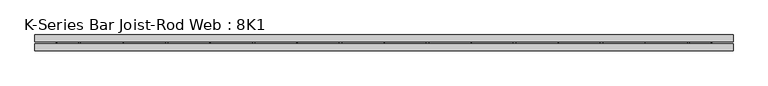
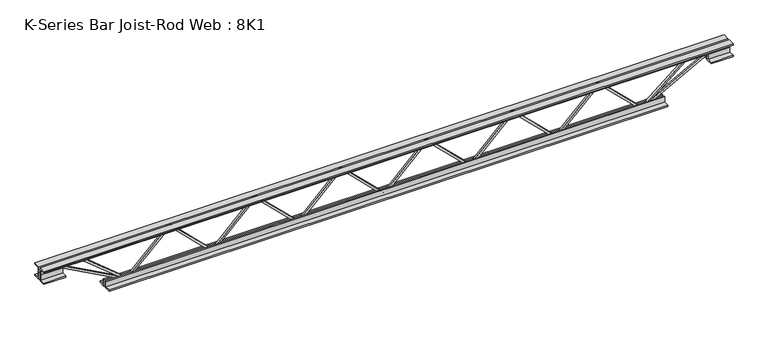
"""IFC4 building model written with IfcOpenShell, lengths in millimetres: beam geometry, K-Series Bar Joist-Rod Web : 8K1."""

from ifc_helpers import new_model, si_unit, frame, origin, place, context, project, spatial, polyline, outline, extrude, source, transform, mapped, element, save


def k_series_bar_joist_rod_web_8k1_a6564055(model_context):
    return source(origin(), model_context, "Body", "SweptSolid", [
        extrude(outline(polyline([(-90.4875, 401.8896924), (-100.0125, 401.8896924), (-100.0125, 407.0077855), (90.4875, 601.6026317), (90.4875, 604.0664455), (-100.0125, 798.6612917), (-100.0125, 803.7793848), (-90.4875, 803.7793848), (-90.4875, 802.5474779), (100.0125, 607.9526317), (100.0125, 597.7164455), (-90.4875, 403.1215993), (-90.4875, 401.8896924)])), frame((0.0, -4.7625, 0.0), z_axis=(0.0, 1.0, 0.0), x_axis=(0.0, 0.0, 1.0)), (0.0, 0.0, 1.0), 9.525),
        extrude(outline(polyline([(-90.4875, 0.0), (-100.0125, 0.0), (-100.0125, 5.1180931), (90.4875, 199.7129393), (90.4875, 202.1767531), (-100.0125, 396.7715993), (-100.0125, 401.8896924), (-90.4875, 401.8896924), (-90.4875, 400.6577855), (100.0125, 206.0629393), (100.0125, 195.8267531), (-90.4875, 1.2319069), (-90.4875, 0.0)])), frame((0.0, -4.7625, 0.0), z_axis=(0.0, 1.0, 0.0), x_axis=(0.0, 0.0, 1.0)), (0.0, 0.0, 1.0), 9.525),
        extrude(outline(polyline([(-90.4875, -401.8896924), (-100.0125, -401.8896924), (-100.0125, -396.7715993), (90.4875, -202.1767531), (90.4875, -199.7129393), (-100.0125, -5.1180931), (-100.0125, 0.0), (-90.4875, 0.0), (-90.4875, -1.2319069), (100.0125, -195.8267531), (100.0125, -206.0629393), (-90.4875, -400.6577855), (-90.4875, -401.8896924)])), frame((0.0, -4.7625, 0.0), z_axis=(0.0, 1.0, 0.0), x_axis=(0.0, 0.0, 1.0)), (0.0, 0.0, 1.0), 9.525),
        extrude(outline(polyline([(-90.4875, -803.7793848), (-100.0125, -803.7793848), (-100.0125, -798.6612917), (90.4875, -604.0664455), (90.4875, -601.6026317), (-100.0125, -407.0077855), (-100.0125, -401.8896924), (-90.4875, -401.8896924), (-90.4875, -403.1215993), (100.0125, -597.7164455), (100.0125, -607.9526317), (-90.4875, -802.5474779), (-90.4875, -803.7793848)])), frame((0.0, -4.7625, 0.0), z_axis=(0.0, 1.0, 0.0), x_axis=(0.0, 0.0, 1.0)), (0.0, 0.0, 1.0), 9.525),
        extrude(outline(polyline([(-90.4875, 803.7793848), (-100.0125, 803.7793848), (-100.0125, 808.8974779), (90.4875, 1003.4923241), (90.4875, 1005.9561379), (-100.0125, 1200.5509841), (-100.0125, 1205.6690772), (-90.4875, 1205.6690772), (-90.4875, 1204.4371703), (100.0125, 1009.8423241), (100.0125, 999.6061379), (-90.4875, 805.0112917), (-90.4875, 803.7793848)])), frame((0.0, -4.7625, 0.0), z_axis=(0.0, 1.0, 0.0), x_axis=(0.0, 0.0, 1.0)), (0.0, 0.0, 1.0), 9.525),
        extrude(outline(polyline([(-90.4875, -1205.6690772), (-100.0125, -1205.6690772), (-100.0125, -1200.5509841), (90.4875, -1005.9561379), (90.4875, -1003.4923241), (-100.0125, -808.8974779), (-100.0125, -803.7793848), (-90.4875, -803.7793848), (-90.4875, -805.0112917), (100.0125, -999.6061379), (100.0125, -1009.8423241), (-90.4875, -1204.4371703), (-90.4875, -1205.6690772)])), frame((0.0, -4.7625, 0.0), z_axis=(0.0, 1.0, 0.0), x_axis=(0.0, 0.0, 1.0)), (0.0, 0.0, 1.0), 9.525),
        extrude(outline(polyline([(4.7625, 101.6), (36.5125, 101.6), (36.5125, 95.25), (11.1125, 95.25), (11.1125, 69.85), (4.7625, 69.85), (4.7625, 101.6)])), frame((-1612.0690772, 0.0, 0.0), z_axis=(1.0, 0.0, 0.0), x_axis=(0.0, 1.0, 0.0)), (0.0, 0.0, 1.0), 3224.1381544),
        extrude(outline(polyline([(-4.7625, 101.6), (-4.7625, 69.85), (-11.1125, 69.85), (-11.1125, 95.25), (-36.5125, 95.25), (-36.5125, 101.6), (-4.7625, 101.6)])), frame((-1612.0690772, 0.0, 0.0), z_axis=(1.0, 0.0, 0.0), x_axis=(0.0, 1.0, 0.0)), (0.0, 0.0, 1.0), 3224.1381544),
        extrude(outline(polyline([(-4.7625, 38.1), (-36.5125, 38.1), (-36.5125, 44.45), (-11.1125, 44.45), (-11.1125, 69.85), (-4.7625, 69.85), (-4.7625, 38.1)])), frame((-1612.0690772, 0.0, 0.0), z_axis=(1.0, 0.0, 0.0), x_axis=(0.0, 1.0, 0.0)), (0.0, 0.0, 1.0), 101.6),
        extrude(outline(polyline([(36.5125, 38.1), (4.7625, 38.1), (4.7625, 69.85), (11.1125, 69.85), (11.1125, 44.45), (36.5125, 44.45), (36.5125, 38.1)])), frame((-1612.0690772, 0.0, 0.0), z_axis=(1.0, 0.0, 0.0), x_axis=(0.0, 1.0, 0.0)), (0.0, 0.0, 1.0), 101.6),
        extrude(outline(polyline([(4.7625, 38.1), (4.7625, 69.85), (11.1125, 69.85), (11.1125, 44.45), (36.5125, 44.45), (36.5125, 38.1), (4.7625, 38.1)])), frame((1510.4690772, 0.0, 0.0), z_axis=(1.0, 0.0, 0.0), x_axis=(0.0, 1.0, 0.0)), (0.0, 0.0, 1.0), 101.6),
        extrude(outline(polyline([(-4.7625, 38.1), (-36.5125, 38.1), (-36.5125, 44.45), (-11.1125, 44.45), (-11.1125, 69.85), (-4.7625, 69.85), (-4.7625, 38.1)])), frame((1510.4690772, 0.0, 0.0), z_axis=(1.0, 0.0, 0.0), x_axis=(0.0, 1.0, 0.0)), (0.0, 0.0, 1.0), 101.6),
        extrude(outline(polyline([(4.7625, -101.6), (4.7625, -69.85), (11.1125, -69.85), (11.1125, -95.25), (36.5125, -95.25), (36.5125, -101.6), (4.7625, -101.6)])), frame((-1307.2690772, 0.0, 0.0), z_axis=(1.0, 0.0, 0.0), x_axis=(0.0, 1.0, 0.0)), (0.0, 0.0, 1.0), 2614.5381544),
        extrude(outline(polyline([(-4.7625, -101.6), (-36.5125, -101.6), (-36.5125, -95.25), (-11.1125, -95.25), (-11.1125, -69.85), (-4.7625, -69.85), (-4.7625, -101.6)])), frame((-1307.2690772, 0.0, 0.0), z_axis=(1.0, 0.0, 0.0), x_axis=(0.0, 1.0, 0.0)), (0.0, 0.0, 1.0), 2614.5381544),
        extrude(outline(polyline([(0.0, -9.525), (0.0, 0.0), (346.6425392, 0.0), (346.6425392, -9.525), (0.0, -9.525)])), frame((-1512.7373757, 4.7625, 65.662372), z_axis=(0.47628314854007997, 0.0, 0.8792919665371384), x_axis=(0.8792919665371384, 0.0, -0.47628314854007997)), (0.0, 0.0, 1.0), 9.525),
        extrude(outline(polyline([(0.0, -9.525), (0.0, 0.0), (260.0708388, 0.0), (260.0708388, -9.525), (0.0, -9.525)])), frame((-1409.6372872, 4.7625, 66.170234), z_axis=(0.6348270368814928, 0.0, 0.7726542779563599), x_axis=(0.7726542779563599, 0.0, -0.6348270368814928)), (0.0, 0.0, 1.0), 9.525),
        extrude(outline(polyline([(0.0, -9.525), (0.0, 0.0), (346.6425392, 0.0), (346.6425392, -9.525), (0.0, -9.525)])), frame((1512.7373757, -4.7625, 65.662372), z_axis=(-0.4762831485400427, 0.0, 0.8792919665371586), x_axis=(-0.8792919665371586, 0.0, -0.4762831485400427)), (0.0, 0.0, 1.0), 9.525),
        extrude(outline(polyline([(0.0, -9.525), (0.0, 0.0), (260.0708388, 0.0), (260.0708388, -9.525), (0.0, -9.525)])), frame((1409.6372872, -4.7625, 66.170234), z_axis=(-0.6348270368814658, 0.0, 0.7726542779563821), x_axis=(-0.7726542779563821, 0.0, -0.6348270368814658)), (0.0, 0.0, 1.0), 9.525),
    ])


if __name__ == "__main__":
    model = new_model("IFC4")
    model_context = context("Model", 3, world=origin())
    ifc_project = project(units=[si_unit("LENGTHUNIT", "METRE", prefix="MILLI")], contexts=[model_context])
    site = spatial("IfcSite", under=ifc_project)
    building = spatial("IfcBuilding", under=site)
    placement = place(None, origin())
    k_series_bar_joist_rod_web_8k1_shape = k_series_bar_joist_rod_web_8k1_a6564055(model_context)
    element("IfcBeam", 1, ObjectType="K-Series Bar Joist-Rod Web : 8K1", at=placement, inside=building, context=model_context, shape_type="MappedRepresentation", body=[
        mapped(k_series_bar_joist_rod_web_8k1_shape, transform((0.0, 0.0, 0.0), x_axis=(1.0, 0.0, 0.0), y_axis=(0.0, 1.0, 0.0), z_axis=(0.0, 0.0, 1.0))),
    ])
    save(model, "model.ifc")

# Revit data of these elements
# Type "K-Series Bar Joist-Rod Web : 8K1"
#   Assembly Code = "B1010350"
#   Wt = 5.1
#   Web Thickness = 0' - 0 3/8"
#   Start Offset [instance default] = 0' - 0"
#   Start Extension [instance default] = 0' - 0"
#   Seat Length = 0' - 4"
#   Seat Depth = 0' - 2 1/2"
#   PanelArrayLength [instance default] = 21' - 4"
#   Panel [instance default] = 1' - 4"
#   End Offset [instance default] = 0' - 0"
#   End Extension [instance default] = 0' - 0"
#   End Panel = 1' - 4"
#   Cord Leg = 0' - 1 1/4"
#   Chord Thickness = 0' - 0 1/4"
#   Length [instance default] = 24' - 0"
#   Depth = 0' - 8"
#   PanelArrayNum [instance default] = 16
#   Rendering Material = none
# Element 1 (IfcBeam, "K-Series Bar Joist-Rod Web : 8K1")
#   PanelArrayLength = 7' - 10.93457"
#   Panel = 1' - 3.82243"
#   PanelArrayNum = 6
